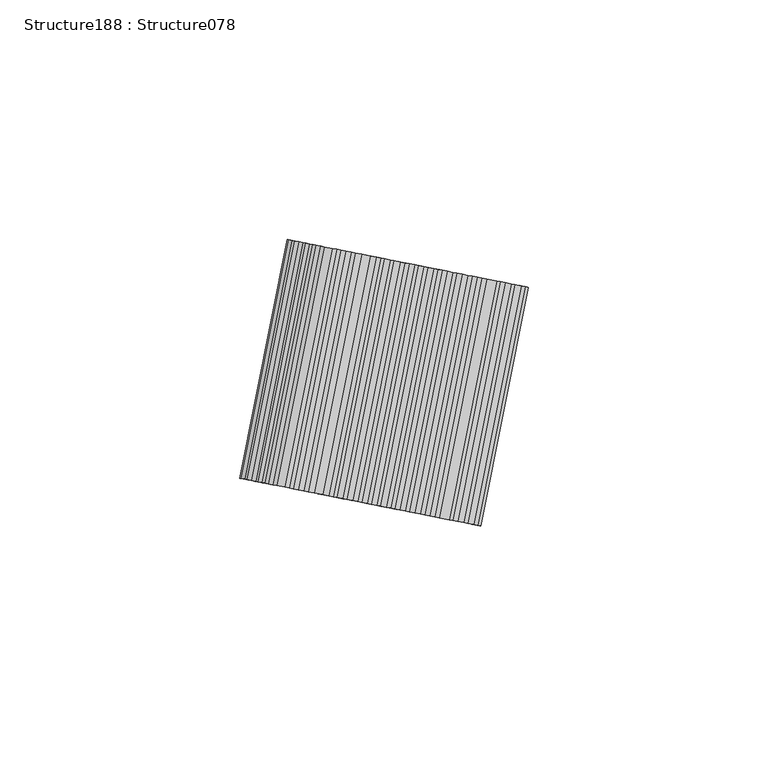
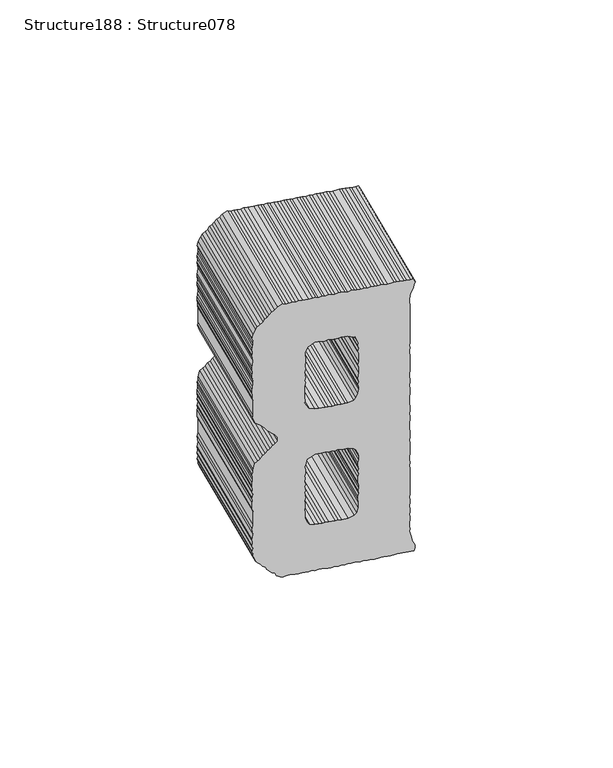
"""IFC4 building model written with IfcOpenShell, lengths in millimetres: proxy geometry, Structure188 : Structure078."""

from ifc_helpers import new_model, si_unit, frame, origin, place, context, project, spatial, polyline, outline, extrude, source, transform, mapped, element, save


def structure188_structure078_5051db7a(model_context):
    return source(origin(), model_context, "Body", "SweptSolid", [
        extrude(outline(polyline([(1.0210831, 0.0), (2.2021055, -0.2015734), (3.2126148, -0.203877), (4.2007987, -0.572012), (5.0440335, -0.3728197), (6.4302813, -0.4104968), (7.4231841, -0.5943601), (8.4067138, -0.9663588), (9.4346593, -0.78077), (11.2137025, -1.5004973), (11.9445593, -2.5830859), (12.504629, -3.4666321), (13.1675905, -4.2652239), (13.7720782, -4.7844835), (14.5344188, -5.5005744), (15.1832292, -6.4843315), (16.5089248, -8.0812414), (17.0724037, -8.9688942), (17.7699069, -9.3979873), (18.3160529, -10.4669725), (19.5597022, -11.9650508), (20.5099353, -12.698578), (21.0906232, -13.3980645), (21.6335873, -14.4632169), (22.5838204, -15.196744), (22.9830828, -15.8798999), (23.909516, -16.7936539), (24.3090057, -17.4770836), (24.9717398, -18.2754016), (25.6204469, -19.2657187), (26.9840934, -20.4972365), (27.4450112, -21.4635573), (28.3918352, -22.1929779), (29.0406456, -23.1767349), (29.8029862, -23.8928259), (30.4657204, -24.691144), (30.8477738, -25.562466), (31.4284617, -26.2619526), (32.2793156, -27.0779806), (32.956428, -27.6914071), (33.6050112, -28.6748905), (34.0832619, -29.4598789), (37.4860245, -33.5587877), (37.0402391, -34.4361665), (36.053481, -35.0819191), (34.8237658, -35.4350096), (33.8746848, -35.7155974), (33.0899701, -36.1936208), (30.8714566, -37.187221), (30.4416351, -37.8844038), (29.4752213, -38.3463239), (28.575334, -39.0933771), (27.9434691, -39.958289), (26.9642732, -40.6042379), (26.1749044, -41.086125), (25.560646, -41.7694772), (24.7628755, -42.4317568), (23.8787818, -42.9922812), (23.0462423, -44.0237857), (22.2443652, -44.6894744), (21.3773305, -45.0688936), (20.7410852, -45.9374419), (19.7618893, -46.5833908), (18.9643925, -47.2454431), (18.4449625, -47.8435981), (17.3631023, -48.5747751), (16.8480527, -49.1692936), (15.8441321, -50.0027113), (14.9629464, -50.5672958), (14.3498866, -51.2431787), (13.3632989, -51.895264), (12.6809748, -52.2882867), (12.0460984, -53.1556986), (10.8822952, -53.781484), (10.1828087, -54.3621718), (9.3662331, -55.2134803), (8.0493064, -56.4736875), (7.0654565, -57.1235001), (6.2679597, -57.7855524), (5.483245, -58.2635759), (4.7487158, -59.2137159), (4.0536096, -59.7907674), (3.1680436, -60.3589882), (2.1829281, -61.0033771), (0.6840285, -62.2477081), (-0.029609, -63.0135612), (-1.0321606, -63.8458425), (-1.8138638, -64.321366), (-2.5486668, -65.2717333), (-3.4325902, -65.8385905), (-5.0148016, -66.9786663), (-6.7110906, -68.3868627), (-7.2303502, -68.9913505), (-8.9266392, -70.3995469), (-9.8142919, -70.9630258), (-10.4458831, -71.8277104), (-11.3257, -72.3911585), (-12.312458, -73.0369109), (-13.1113236, -73.7000996), (-13.7285935, -74.3859518), (-14.5436968, -75.2295638), (-16.1447133, -76.5586686), (-16.8241292, -76.9557512), (-17.7418969, -77.8845914), (-19.3078706, -78.8442439), (-20.1447904, -79.8793848), (-21.0088136, -80.256304), (-21.623072, -80.9396562), (-22.5408397, -81.8684963), (-23.2243622, -82.2689882), (-24.0391917, -83.1123728), (-25.7384923, -84.5230693), (-26.5244054, -85.008562), (-28.2190517, -86.4153948), (-28.8414198, -87.0990052), (-29.8203419, -87.7447267), (-30.3397719, -88.3428817), (-32.0346921, -89.7499417), (-32.9061071, -90.1329973), (-33.9056473, -90.9627786), (-35.1517706, -92.5110427), (-35.4995922, -93.3075582), (-35.9701022, -94.372406), (-36.6871953, -95.1346535), (-37.1533249, -96.1958648), (-38.4729224, -96.4501548), (-38.9498043, -95.6640299), (-39.7798128, -94.664216), (-40.3827149, -94.1496518), (-41.2129508, -93.1495641), (-41.9736952, -92.4326106), (-42.472564, -91.8316818), (-43.5962161, -90.0670429), (-44.2623593, -89.2646183), (-45.127137, -88.6340292), (-45.69527, -87.7502401), (-46.2759578, -87.0507536), (-47.1189758, -86.2346948), (-47.6651219, -85.1657095), (-48.349843, -84.5525875), (-48.9908175, -83.5687997), (-49.760994, -82.8527396), (-50.3416818, -82.153253), (-51.0206072, -81.5348573), (-51.6487996, -80.3670405), (-52.2482925, -79.8565829), (-53.0944923, -79.0366913), (-53.5931339, -78.4360363), (-54.2433132, -77.4534156), (-54.824001, -76.7539291), (-55.5849727, -76.0367018), (-56.3171983, -74.9552495), (-56.9106683, -74.4397919), (-57.5388607, -73.2719751), (-58.239773, -72.8387755), (-58.8204608, -72.1392889), (-59.5558683, -71.0540039), (-60.7142894, -69.6585899), (-61.6425356, -68.7398667), (-62.0211799, -67.8726512), (-62.8702208, -67.0615923), (-63.5363641, -66.2591677), (-64.0130187, -65.4733167), (-64.7959774, -64.9412854), (-65.2754266, -63.1426832), (-65.156628, -61.8625088), (-65.3378365, -60.830927), (-65.1326112, -59.6459478), (-64.9488821, -58.6517692), (-65.14747, -57.8020207), (-64.6801987, -56.7393993), (-64.7587893, -55.6230903), (-64.8422615, -54.5103712), (-64.4770501, -53.5264642), (-63.7711534, -51.9318579), (-62.9418992, -50.9030808), (-62.0721267, -50.5213888), (-61.1749771, -49.7766083), (-60.6555471, -49.1784534), (-59.9383507, -48.4096458), (-58.8565938, -47.6850288), (-58.1440514, -46.9200849), (-57.3549565, -46.438425), (-56.3757606, -45.7924761), (-54.9420185, -44.2618755), (-54.242532, -43.6811877), (-53.255774, -43.0354352), (-52.6412418, -42.3518557), (-51.9417553, -41.7711678), (-50.8773312, -41.2278833), (-50.0795608, -40.5656037), (-49.2600771, -39.7183553), (-48.5431544, -38.949775), (-47.7442888, -38.2865863), (-46.9593003, -37.8083355), (-46.0624246, -37.0637823), (-45.2806179, -36.5816987), (-41.1814354, -33.1787089), (-40.56071, -32.4964623), (-38.7461799, -31.8317599), (-37.5862765, -32.2173465), (-36.5850367, -32.4012254), (-35.5919637, -32.5914215), (-34.3905969, -32.6091624), (-33.2774232, -32.5262378), (-32.4608941, -32.6965134), (-31.4636111, -32.8767403), (-30.2003719, -33.183478), (-28.9848077, -33.0155526), (-27.8858884, -32.1032704), (-27.7022058, -31.1095928), (-27.7983566, -30.1743424), (-27.6825694, -28.8966682), (-27.6793411, -27.878917), (-27.4753143, -26.701407), (-27.579301, -25.7661875), (-27.2756213, -24.5059494), (-27.3720458, -23.5709263), (-27.3509837, -22.3718891), (-26.1809407, -20.7258525), (-25.3820751, -20.0626638), (-24.9519798, -19.3652536), (-24.0648746, -18.8022293), (-23.2671041, -18.1399497), (-22.5504552, -17.3715967), (-21.6516629, -16.6254525), (-20.768938, -16.0660645), (-20.0520153, -15.2974842), (-19.1882659, -14.9207923), (-18.4540103, -13.9708795), (-17.5666313, -13.4076279), (-17.0547636, -12.8092766), (-15.2530725, -11.3135793), (-14.3893231, -10.9368874), (-10.5912893, -7.7839001), (-9.7543694, -6.7487592), (-7.9904589, -5.6247868), (-6.8567706, -4.3432797), (-5.9737719, -3.7836645), (-5.0594599, -2.8512188), (-4.0930461, -2.3892987), (-3.4581696, -1.5218868), (-2.5914087, -1.1426948), (-1.8919222, -0.562007), (0.0, 0.0), (1.0210831, 0.0)]), holes=[polyline([(-32.0402526, -47.0360164), (-32.9248939, -47.5969952), (-33.9244341, -48.4267766), (-35.3234071, -49.5881523), (-36.125558, -50.2540682), (-36.8565747, -51.2017548), (-37.6195297, -51.4943084), (-38.2558214, -52.3633578), (-40.0199593, -53.4870563), (-40.6546085, -54.3547421), (-41.6340317, -55.0004172), (-43.0533954, -56.3461264), (-43.7531557, -56.9270415), (-44.6342948, -57.4911248), (-45.5358248, -58.2395417), (-46.2341594, -59.8343443), (-45.8262315, -62.3600944), (-45.2421345, -63.0636874), (-44.4811163, -63.7804138), (-43.6367295, -64.5953362), (-43.2502956, -65.4630219), (-42.2255785, -66.2951843), (-40.8967011, -67.895927), (-40.5957226, -68.6606746), (-39.9327612, -69.4592663), (-39.1715158, -70.1762664), (-37.4052548, -71.0800226), (-36.4079716, -71.2602495), (-34.7938993, -70.7679717), (-34.0802619, -70.0021187), (-33.1149896, -69.5416087), (-32.4806142, -68.6741503), (-31.7157429, -68.3800058), (-29.3125755, -66.3849851), (-28.6809379, -65.5197995), (-27.81833, -65.1445176), (-26.3166927, -63.8979138), (-24.883178, -62.3670395), (-23.8185267, -61.8240287), (-23.2818877, -61.0377075), (-22.2175102, -60.494924), (-21.6160339, -59.9956006), (-20.7837216, -58.9638224), (-20.097942, -57.5533223), (-19.9142595, -56.5596447), (-20.6763262, -54.8222436), (-21.2540595, -54.126316), (-21.9031437, -53.1427864), (-22.5658779, -52.3444683), (-23.2490802, -51.7231488), (-23.7306627, -50.9413887), (-24.656822, -50.0274073), (-25.1418137, -49.2415407), (-26.6692789, -47.8121325), (-27.4174685, -46.9108763), (-28.9917305, -46.0211472), (-31.4232566, -46.3503914), (-32.0402526, -47.0360164)]), polyline([(-14.9308199, -34.6886598), (-14.5537612, -36.572263), (-13.9525018, -37.0881908), (-13.2897676, -37.8865088), (-12.6471505, -38.8689331), (-11.960663, -39.4875253), (-11.2158825, -40.3846749), (-10.4549109, -41.1019023), (-10.0712147, -41.9718607), (-9.0439871, -42.8014765), (-7.7969288, -44.3036614), (-6.3179394, -45.2724823), (-5.5048194, -45.4386512), (-3.8045942, -45.0417958), (-2.9231812, -44.4774851), (-2.0230201, -43.7302047), (-1.3886448, -42.8627463), (-0.6918959, -42.2843312), (0.475146, -41.6563195), (1.0071307, -40.873862), (1.8743927, -40.4947166), (2.5087681, -39.6272582), (4.0076677, -38.3829271), (5.0766994, -37.8362799), (5.8741961, -37.1742276), (6.4886713, -36.4967072), (7.2748118, -36.0114883), (7.9050805, -35.1474391), (8.7069577, -34.4817503), (9.6893354, -33.8396342), (11.2906256, -32.5103022), (12.2570394, -31.0272991), (12.3586757, -29.9347901), (11.6991699, -28.1187208), (10.3700652, -26.5177044), (9.5052876, -25.8871153), (8.9418087, -24.9994625), (7.6981594, -23.5013842), (6.8473055, -22.6853561), (6.4718429, -21.8219735), (5.7063206, -21.1020497), (4.7734203, -20.1871901), (3.4790381, -19.2385327), (2.6485854, -19.2536962), (0.7507436, -19.8141432), (-0.7465134, -21.0571107), (-1.7332716, -21.7028631), (-2.4501942, -22.4714435), (-3.2493336, -23.1348595), (-4.1364389, -23.6978838), (-4.7680764, -24.5630695), (-5.5454562, -25.0410156), (-6.5322143, -25.686768), (-6.96482, -26.3867247), (-8.031114, -26.9310991), (-8.5661102, -27.7160567), (-9.5327513, -28.1777029), (-10.3474105, -29.0274206), (-11.0297346, -29.4204431), (-11.6657525, -30.2892652), (-12.6655665, -31.1192738), (-13.630565, -31.5795564), (-14.0645395, -32.2806495), (-15.1292373, -33.8452442), (-14.9308199, -34.6886598)])]), frame((-2997.9941383, 235063.4558145, 394.0690536), z_axis=(0.19466222296394123, 0.9808703374813295, 0.0), x_axis=(0.6265247473504413, -0.12433926830158984, -0.7694195781988465)), (0.0, 0.0, 1.0), 50.8),
    ])


if __name__ == "__main__":
    model = new_model("IFC4")
    model_context = context("Model", 3, world=origin())
    ifc_project = project(units=[si_unit("LENGTHUNIT", "METRE", prefix="MILLI")], contexts=[model_context])
    site = spatial("IfcSite", under=ifc_project)
    building = spatial("IfcBuilding", under=site)
    placement = place(None, origin())
    structure188_structure078_shape = structure188_structure078_5051db7a(model_context)
    element("IfcBuildingElementProxy", 1, Name="Structure188 : Structure078", ObjectType="Structure188 : Structure078", at=placement, inside=building, context=model_context, shape_type="MappedRepresentation", body=[
        mapped(structure188_structure078_shape, transform((0.0, 0.0, 0.0), x_axis=(1.0, 0.0, 0.0), y_axis=(0.0, 1.0, 0.0), z_axis=(0.0, 0.0, 1.0))),
    ])
    save(model, "model.ifc")

# Revit data of these elements
# Type "Structure188 : Structure078"
#   NameOverride = "Structure078"
# Element 1 (IfcBuildingElementProxy, "Structure188 : Structure078")
#   Materials on its faces: "BRUSHED ALUMINUM LETTERING"
# Materials
#   "BRUSHED ALUMINUM LETTERING": class "Unassigned", colour RGB 169 181 186, transparency 0, Cost = 0
